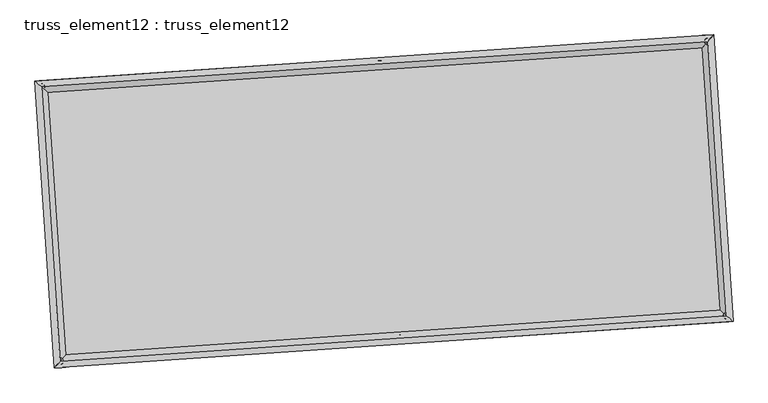
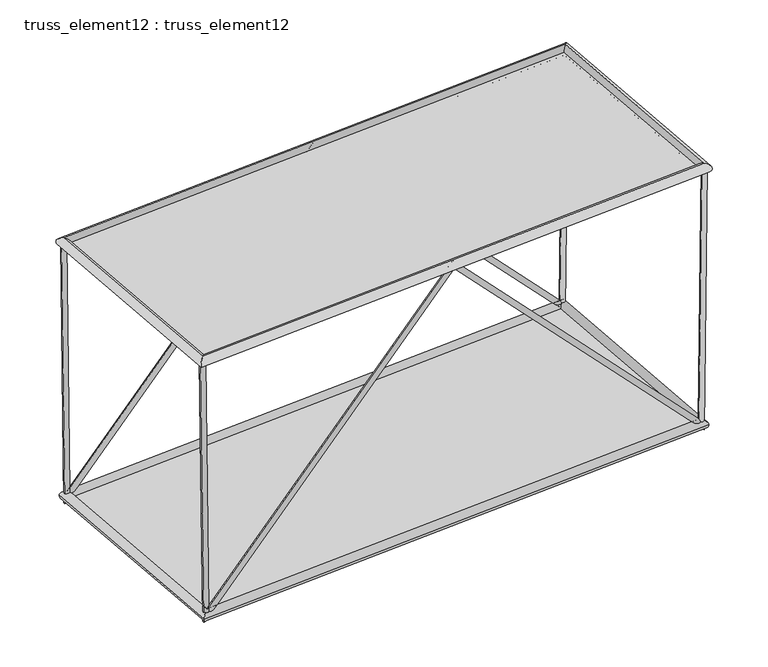
"""IFC4 building model written with IfcOpenShell, lengths in millimetres: plate geometry, truss_element12 : truss_element12."""

from ifc_helpers import new_model, si_unit, frame, origin, origin_with_axes, place, context, project, spatial, polyline, circle_curve, ellipse_curve, outline, extrude, source, transform, mapped, element, save
from ifc_brep_helpers import plane_surface, cylinder_surface, advanced_brep


def truss_element12_truss_element12_2c86acb7(model_context):
    return source(origin(), model_context, "Body", "SolidModel", [
        advanced_brep(
        [(-3728.3550112, 2271.9000693, 5000.230225), (-3827.45033, 2258.5393422, 4998.9618576), (-3666.4925131, 2276.1182379, 122.5885244), (-3762.4943697, 2262.9684422, -122.5885244), (1063.1473442, 2598.6144007, 5071.7241818), (1063.6040901, 2592.0417504, 4927.4822409), (5793.903749, 2921.1866967, 122.5964773), (5890.857228, 2921.1937918, -122.5964773), (5854.658099, 2925.3293049, 5000.2332074), (5954.6501108, 2925.543586, 4998.9875555)],
        [
            (0, 1, circle_curve(frame((-3777.9026706, 2265.2197058, 4999.5960413), z_axis=(-0.012681845830498275, -0.0008647268589742656, 0.9999192082532422), x_axis=(-0.13360744533254773, 0.991033979828119, -0.0008374829847137765)), 50.0)),
            (1, 0, circle_curve(frame((-3777.9026706, 2265.2197058, 4999.5960413), z_axis=(-0.012681845830498275, -0.0008647268589742656, 0.9999192082532422), x_axis=(-0.13360744533254773, 0.991033979828119, -0.0008374829847137765)), 50.0)),
            (0, 2),
            (2, 3, ellipse_curve(frame((-3714.4934414, 2269.54334, 0.0), z_axis=(-0.9281379125811652, -0.06328619607639939, 0.3668172196280557), x_axis=(0.36596744941726267, 0.02495392920324594, 0.9302930330730971)), 132.0610358, 50.0)),
            (3, 1),
            (3, 2, ellipse_curve(frame((-3714.4934414, 2269.54334, 0.0), z_axis=(-0.9281379125811652, -0.06328619607639939, 0.3668172196280557), x_axis=(0.36596744941726267, 0.02495392920324594, 0.9302930330730971)), 132.0610358, 50.0)),
            (2, 4),
            (4, 5, ellipse_curve(frame((1063.3757172, 2595.3280756, 4999.6032114), z_axis=(-0.99768339431723, -0.068028238108855, -5.9358703528731525e-05), x_axis=(5.922119292306359e-05, 4.038068026292035e-06, -0.9999999982382721)), 72.2780144, 50.0)),
            (5, 3),
            (5, 4, ellipse_curve(frame((1063.3757172, 2595.3280756, 4999.6032114), z_axis=(-0.99768339431723, -0.068028238108855, -5.9358703528731525e-05), x_axis=(5.922119292306359e-05, 4.038068026292035e-06, -0.9999999982382721)), 72.2780144, 50.0)),
            (4, 6),
            (6, 7, ellipse_curve(frame((5842.3804885, 2921.1902443, 0.0), z_axis=(-0.9280745157714422, -0.06328187328893672, -0.3669783340861503), x_axis=(-0.3661281906369709, -0.02496488953598652, 0.9302294890570573)), 132.0786249, 50.0)),
            (7, 5),
            (7, 6, ellipse_curve(frame((5842.3804885, 2921.1902443, 0.0), z_axis=(-0.9280745157714422, -0.06328187328893672, -0.3669783340861503), x_axis=(-0.3661281906369709, -0.02496488953598652, 0.9302294890570573)), 132.0786249, 50.0)),
            (8, 9, circle_curve(frame((5904.6541049, 2925.4364454, 4999.6103815), z_axis=(0.012454723282468173, 0.0008492402357941579, 0.9999220762934375), x_axis=(-0.002153222592044798, 0.9999973435725115, -0.0008224842793232085)), 50.0)),
            (9, 8, circle_curve(frame((5904.6541049, 2925.4364454, 4999.6103815), z_axis=(0.012454723282468173, 0.0008492402357941579, 0.9999220762934375), x_axis=(-0.002153222592044798, 0.9999973435725115, -0.0008224842793232085)), 50.0)),
            (6, 8),
            (9, 7),
        ],
        [
            plane_surface(frame((-3777.9026706, 2315.2196871, 4999.6392811), z_axis=(-0.012681845830499536, -0.000864726858973905, 0.9999192082532424), x_axis=(0.9999195821596513, -1.0967214670642997e-05, 0.012681841088294742))),
            cylinder_surface(frame((-3777.9026706, 2265.2197058, 4999.5960413), z_axis=(-0.012681845830498278, -0.0008647268589742659, 0.9999192082532424), x_axis=(-0.13360744533254773, 0.991033979828119, -0.0008374829847137765)), 50.0),
            cylinder_surface(frame((-3714.4934414, 2269.54334, 0.0), z_axis=(-0.6901279623524452, -0.04705720233082468, -0.7221558109494499), x_axis=(-0.020411445780293115, 0.9987523847393089, -0.04557462955089897)), 50.0),
            cylinder_surface(frame((1063.3757172, 2595.3280756, 4999.6032114), z_axis=(-0.6902134913462256, -0.04706303422778687, 0.7220736854178583), x_axis=(-0.11534401236489931, 0.9922792938963748, -0.04558027770953044)), 50.0),
            plane_surface(frame((5904.6541049, 2875.4364635, 4999.6528468), z_axis=(0.012454723282466664, 0.0008492402357928526, 0.9999220762934377), x_axis=(0.9999224369259634, -1.0577872590289415e-05, -0.012454718790539939))),
            cylinder_surface(frame((5842.3804885, 2921.1902443, 0.0), z_axis=(-0.012454723282468173, -0.0008492402357941579, -0.9999220762934375), x_axis=(-0.002153222592044798, 0.9999973435725115, -0.0008224842793232085)), 50.0),
        ],
        [
            (0, [[1, 2]]),
            (1, [[-1, 3, 4, 5]]),
            (1, [[-2, -5, 6, -3]]),
            (2, [[-4, 7, 8, 9]]),
            (2, [[-6, -9, 10, -7]]),
            (3, [[-8, 11, 12, 13]]),
            (3, [[-10, -13, 14, -11]]),
            (4, [[15, 16]]),
            (5, [[-12, 17, -16, 18]]),
            (5, [[-14, -18, -15, -17]]),
        ],
    ),
        advanced_brep(
        [(-3456.2420582, -1718.833515, 5000.230225), (-3555.3373771, -1732.1942421, 4998.9618576), (-3394.3795602, -1714.6153464, 122.5885244), (-3490.3814168, -1727.7651421, -122.5885244), (1335.2602971, -1392.1191836, 5071.7241818), (1335.7170431, -1398.6918339, 4927.4822409), (6066.016702, -1069.5468876, 122.5964773), (6162.9701809, -1069.5397925, -122.5964773), (6126.7710519, -1065.4042794, 5000.2332074), (6226.7630638, -1065.1899983, 4998.9875555)],
        [
            (0, 1, circle_curve(frame((-3505.7897177, -1725.5138785, 4999.5960413), z_axis=(-0.012681845830497715, -0.0008647268589742125, 0.9999192082532423), x_axis=(-0.13360744533254784, 0.991033979828119, -0.0008374829847137556)), 50.0)),
            (1, 0, circle_curve(frame((-3505.7897177, -1725.5138785, 4999.5960413), z_axis=(-0.012681845830497715, -0.0008647268589742125, 0.9999192082532423), x_axis=(-0.13360744533254784, 0.991033979828119, -0.0008374829847137556)), 50.0)),
            (0, 2),
            (2, 3, ellipse_curve(frame((-3442.3804885, -1721.1902443, 0.0), z_axis=(-0.9281379125811646, -0.06328619607639936, 0.36681721962805663), x_axis=(0.3659674494172635, 0.02495392920324602, 0.930293033073097)), 132.0610358, 50.0)),
            (3, 1),
            (3, 2, ellipse_curve(frame((-3442.3804885, -1721.1902443, 0.0), z_axis=(-0.9281379125811646, -0.06328619607639936, 0.36681721962805663), x_axis=(0.3659674494172635, 0.02495392920324602, 0.930293033073097)), 132.0610358, 50.0)),
            (2, 4),
            (4, 5, ellipse_curve(frame((1335.4886701, -1395.4055087, 4999.6032114), z_axis=(-0.9976833943172299, -0.06802823810885503, -5.935870352808952e-05), x_axis=(5.922119292244865e-05, 4.03806802626321e-06, -0.9999999982382721)), 72.2780144, 50.0)),
            (5, 3),
            (5, 4, ellipse_curve(frame((1335.4886701, -1395.4055087, 4999.6032114), z_axis=(-0.9976833943172299, -0.06802823810885503, -5.935870352808952e-05), x_axis=(5.922119292244865e-05, 4.03806802626321e-06, -0.9999999982382721)), 72.2780144, 50.0)),
            (4, 6),
            (6, 7, ellipse_curve(frame((6114.4934414, -1069.54334, 0.0), z_axis=(-0.928074515771442, -0.06328187328893677, -0.3669783340861506), x_axis=(-0.3661281906369714, -0.024964889535986565, 0.9302294890570572)), 132.0786249, 50.0)),
            (7, 5),
            (7, 6, ellipse_curve(frame((6114.4934414, -1069.54334, 0.0), z_axis=(-0.928074515771442, -0.06328187328893677, -0.3669783340861506), x_axis=(-0.3661281906369714, -0.024964889535986565, 0.9302294890570572)), 132.0786249, 50.0)),
            (8, 9, circle_curve(frame((6176.7670578, -1065.2971389, 4999.6103815), z_axis=(0.012454723282467507, 0.0008492402357941209, 0.9999220762934375), x_axis=(-0.0021532225920447086, 0.9999973435725115, -0.0008224842793231741)), 50.0)),
            (9, 8, circle_curve(frame((6176.7670578, -1065.2971389, 4999.6103815), z_axis=(0.012454723282467507, 0.0008492402357941209, 0.9999220762934375), x_axis=(-0.0021532225920447086, 0.9999973435725115, -0.0008224842793231741)), 50.0)),
            (6, 8),
            (9, 7),
        ],
        [
            plane_surface(frame((-3505.7897177, -1675.5138972, 4999.6392811), z_axis=(-0.012681845830499536, -0.000864726858973898, 0.9999192082532424), x_axis=(0.9999195821596513, -1.0967214670642997e-05, 0.012681841088294742))),
            cylinder_surface(frame((-3505.7897177, -1725.5138785, 4999.5960413), z_axis=(-0.012681845830497715, -0.0008647268589742125, 0.9999192082532423), x_axis=(-0.13360744533254784, 0.991033979828119, -0.0008374829847137556)), 50.0),
            cylinder_surface(frame((-3442.3804885, -1721.1902443, 0.0), z_axis=(-0.6901279623524461, -0.047057202330824756, -0.722155810949449), x_axis=(-0.020411445780293143, 0.9987523847393089, -0.045574629550899075)), 50.0),
            cylinder_surface(frame((1335.4886701, -1395.4055087, 4999.6032114), z_axis=(-0.6902134913462256, -0.047063034227786904, 0.7220736854178583), x_axis=(-0.11534401236489945, 0.9922792938963748, -0.045580277709530506)), 50.0),
            plane_surface(frame((6176.7670578, -1115.2971208, 4999.6528468), z_axis=(0.012454723282466664, 0.0008492402357928471, 0.9999220762934377), x_axis=(0.9999224369259634, -1.0577872589401237e-05, -0.012454718790539939))),
            cylinder_surface(frame((6114.4934414, -1069.54334, 0.0), z_axis=(-0.012454723282467507, -0.0008492402357941209, -0.9999220762934375), x_axis=(-0.0021532225920447086, 0.9999973435725115, -0.0008224842793231741)), 50.0),
        ],
        [
            (0, [[1, 2]]),
            (1, [[-1, 3, 4, 5]]),
            (1, [[-2, -5, 6, -3]]),
            (2, [[-4, 7, 8, 9]]),
            (2, [[-6, -9, 10, -7]]),
            (3, [[-8, 11, 12, 13]]),
            (3, [[-10, -13, 14, -11]]),
            (4, [[15, 16]]),
            (5, [[-12, 17, -16, 18]]),
            (5, [[-14, -18, -15, -17]]),
        ],
    ),
        advanced_brep(
        [(-3505.7859545, -1725.5097077, 4909.5960414), (-3505.7934808, -1725.5180494, 5089.5960412), (-3777.906965, 2265.2233272, 5089.5960412), (-3777.8983761, 2265.2160844, 4909.5960414), (5904.6576027, 2925.4405981, 5089.6103814), (5904.6506071, 2925.4322927, 4909.6103815), (6176.7710869, -1065.3007784, 5089.6103814), (6176.7630287, -1065.2934994, 4909.6103815)],
        [
            (0, 1, ellipse_curve(frame((-3505.7897177, -1725.5138785, 4999.5960413), z_axis=(-0.7535719234046869, 0.6573654662781344, -1.0448234971291915e-06), x_axis=(-0.6573654662773117, -0.7535719234054046, -1.0448235032548692e-06)), 127.2792206, 90.0)),
            (1, 2),
            (2, 3, ellipse_curve(frame((-3777.9026706, 2265.2197058, 4999.5960413), z_axis=(-0.6573654662773116, -0.7535719234054046, -1.0448235045172827e-06), x_axis=(0.7535719234046869, -0.6573654662781343, 1.0448234983916052e-06)), 127.2792206, 90.0)),
            (3, 0),
            (1, 0, ellipse_curve(frame((-3505.7897177, -1725.5138785, 4999.5960413), z_axis=(-0.7535719234046869, 0.6573654662781344, -1.0448234971291915e-06), x_axis=(-0.6573654662773117, -0.7535719234054046, -1.0448235032548692e-06)), 127.2792206, 90.0)),
            (3, 2, ellipse_curve(frame((-3777.9026706, 2265.2197058, 4999.5960413), z_axis=(-0.6573654662773116, -0.7535719234054046, -1.0448235045172827e-06), x_axis=(0.7535719234046869, -0.6573654662781343, 1.0448234983916052e-06)), 127.2792206, 90.0)),
            (2, 4),
            (4, 5, ellipse_curve(frame((5904.6541049, 2925.4364454, 4999.6103815), z_axis=(-0.7535719234046876, 0.6573654662781336, -1.0448234953288471e-06), x_axis=(-0.6573654662773109, -0.7535719234054052, -1.0448235075800405e-06)), 127.2792206, 90.0)),
            (5, 3),
            (5, 4, ellipse_curve(frame((5904.6541049, 2925.4364454, 4999.6103815), z_axis=(-0.7535719234046876, 0.6573654662781336, -1.0448234953288471e-06), x_axis=(-0.6573654662773109, -0.7535719234054052, -1.0448235075800405e-06)), 127.2792206, 90.0)),
            (4, 6),
            (6, 7, ellipse_curve(frame((6176.7670578, -1065.2971389, 4999.6103815), z_axis=(0.657365466277311, 0.753571923405405, 1.044823506317627e-06), x_axis=(-0.7535719234046873, 0.6573654662781341, -1.0448234940664328e-06)), 127.2792206, 90.0)),
            (7, 5),
            (7, 6, ellipse_curve(frame((6176.7670578, -1065.2971389, 4999.6103815), z_axis=(0.657365466277311, 0.753571923405405, 1.044823506317627e-06), x_axis=(-0.7535719234046873, 0.6573654662781341, -1.0448234940664328e-06)), 127.2792206, 90.0)),
            (6, 1),
            (0, 7),
        ],
        [
            cylinder_surface(frame((-3505.7897177, -1725.5138785, 4999.5960413), z_axis=(0.06802823822869937, -0.9976833960748767, 0.0), x_axis=(-0.997683395070632, -0.06802823816022374, -4.486817461283446e-05)), 90.0),
            cylinder_surface(frame((-3777.9026706, 2265.2197058, 4999.5960413), z_axis=(-0.9976833960737876, -0.06802823822862634, -1.47760356604302e-06), x_axis=(-0.06802823810069528, 0.9976833951400482, -4.339057104385098e-05)), 90.0),
            cylinder_surface(frame((5904.6541049, 2925.4364454, 4999.6103815), z_axis=(-0.06802823822870101, 0.9976833960748767, 0.0), x_axis=(0.997683395198563, 0.06802823816894851, -4.19129674878619e-05)), 90.0),
            cylinder_surface(frame((6176.7670578, -1065.2971389, 4999.6103815), z_axis=(0.9976833960737875, 0.06802823822862625, 1.4776035642576973e-06), x_axis=(0.06802823822862625, -0.997683395131325, -4.339057105939159e-05)), 90.0),
        ],
        [
            (0, [[1, 2, 3, 4]]),
            (0, [[5, -4, 6, -2]]),
            (1, [[-3, 7, 8, 9]]),
            (1, [[-6, -9, 10, -7]]),
            (2, [[-8, 11, 12, 13]]),
            (2, [[-10, -13, 14, -11]]),
            (3, [[-12, 15, -1, 16]]),
            (3, [[-14, -16, -5, -15]]),
        ],
    ),
        advanced_brep(
        [(-3358.7115243, -1625.2761972, 0.0), (-3526.0494527, -1817.1042913, 0.0), (-3810.4074885, 2353.2123043, 0.0), (-3618.5793943, 2185.8743758, 0.0), (5926.0494527, 3017.1042913, 0.0), (5758.7115243, 2825.2761972, 0.0), (6210.4074885, -1153.2123043, 0.0), (6018.5793943, -985.8743758, 0.0)],
        [
            (0, 1, ellipse_curve(frame((-3442.3804885, -1721.1902443, 0.0), z_axis=(-0.753571923405458, 0.6573654662780806, 0.0), x_axis=(-0.6573654662780806, -0.753571923405458, 0.0)), 127.2792206, 90.0)),
            (1, 2),
            (2, 3, ellipse_curve(frame((-3714.4934414, 2269.54334, 0.0), z_axis=(-0.6573654662780806, -0.753571923405458, 0.0), x_axis=(0.7535719234054579, -0.6573654662780809, 0.0)), 127.2792206, 90.0)),
            (3, 0),
            (1, 0, ellipse_curve(frame((-3442.3804885, -1721.1902443, 0.0), z_axis=(-0.753571923405458, 0.6573654662780806, 0.0), x_axis=(-0.6573654662780806, -0.753571923405458, 0.0)), 127.2792206, 90.0)),
            (3, 2, ellipse_curve(frame((-3714.4934414, 2269.54334, 0.0), z_axis=(-0.6573654662780806, -0.753571923405458, 0.0), x_axis=(0.7535719234054579, -0.6573654662780809, 0.0)), 127.2792206, 90.0)),
            (2, 4),
            (4, 5, ellipse_curve(frame((5842.3804885, 2921.1902443, 0.0), z_axis=(-0.7535719234054586, 0.6573654662780799, 0.0), x_axis=(-0.6573654662780801, -0.7535719234054584, 0.0)), 127.2792206, 90.0)),
            (5, 3),
            (5, 4, ellipse_curve(frame((5842.3804885, 2921.1902443, 0.0), z_axis=(-0.7535719234054586, 0.6573654662780799, 0.0), x_axis=(-0.6573654662780801, -0.7535719234054584, 0.0)), 127.2792206, 90.0)),
            (4, 6),
            (6, 7, ellipse_curve(frame((6114.4934414, -1069.54334, 0.0), z_axis=(0.6573654662780799, 0.7535719234054586, 0.0), x_axis=(-0.7535719234054586, 0.6573654662780799, 0.0)), 127.2792206, 90.0)),
            (7, 5),
            (7, 6, ellipse_curve(frame((6114.4934414, -1069.54334, 0.0), z_axis=(0.6573654662780799, 0.7535719234054586, 0.0), x_axis=(-0.7535719234054586, 0.6573654662780799, 0.0)), 127.2792206, 90.0)),
            (6, 1),
            (0, 7),
        ],
        [
            cylinder_surface(frame((-3442.3804885, -1721.1902443, 0.0), z_axis=(0.06802823822870088, -0.9976833960748768, 0.0), x_axis=(-0.9976833960748768, -0.06802823822870088, 0.0)), 90.0),
            cylinder_surface(frame((-3714.4934414, 2269.54334, 0.0), z_axis=(-0.9976833960748767, -0.06802823822870208, 0.0), x_axis=(-0.06802823822870208, 0.9976833960748767, 0.0)), 90.0),
            cylinder_surface(frame((5842.3804885, 2921.1902443, 0.0), z_axis=(-0.06802823822870274, 0.9976833960748765, 0.0), x_axis=(0.9976833960748765, 0.06802823822870274, 0.0)), 90.0),
            cylinder_surface(frame((6114.4934414, -1069.54334, 0.0), z_axis=(0.9976833960748767, 0.06802823822870205, 0.0), x_axis=(0.06802823822870205, -0.9976833960748767, 0.0)), 90.0),
        ],
        [
            (0, [[1, 2, 3, 4]]),
            (0, [[5, -4, 6, -2]]),
            (1, [[-3, 7, 8, 9]]),
            (1, [[-6, -9, 10, -7]]),
            (2, [[-8, 11, 12, 13]]),
            (2, [[-10, -13, 14, -11]]),
            (3, [[-12, 15, -1, 16]]),
            (3, [[-14, -16, -5, -15]]),
        ],
    ),
        extrude(outline(polyline([(-3442.3804885, -1721.1902443), (-3714.4934414, 2269.54334), (5842.3804885, 2921.1902443), (6114.4934414, -1069.54334), (-3442.3804885, -1721.1902443)])), origin_with_axes(), (0.0, 0.0, 1.0), 20.0),
        extrude(outline(polyline([(-1999.9999999, 4852.5197541), (2000.0000001, 4852.5197541), (2000.0, -4852.5197541), (-2000.0, -4852.5197541), (-1999.9999999, 4852.5197541)])), frame((1199.4321936, 599.9612834, 4999.6032114), z_axis=(-1.474180543527448e-06, -1.0051877171978412e-07, 0.9999999999989084), x_axis=(-0.06802823822870088, 0.9976833960748767, 0.0)), (0.0, 0.0, 1.0), 20.0),
    ])


if __name__ == "__main__":
    model = new_model("IFC4")
    model_context = context("Model", 3, world=origin())
    ifc_project = project(units=[si_unit("LENGTHUNIT", "METRE", prefix="MILLI")], contexts=[model_context])
    site = spatial("IfcSite", under=ifc_project)
    building = spatial("IfcBuilding", under=site)
    placement = place(None, origin())
    truss_element12_truss_element12_shape = truss_element12_truss_element12_2c86acb7(model_context)
    element("IfcPlate", 1, ObjectType="truss_element12 : truss_element12", at=placement, inside=building, context=model_context, shape_type="MappedRepresentation", body=[
        mapped(truss_element12_truss_element12_shape, transform((0.0, 0.0, 0.0), x_axis=(1.0, 0.0, 0.0), y_axis=(0.0, 1.0, 0.0), z_axis=(0.0, 0.0, 1.0))),
    ])
    save(model, "model.ifc")

# Revit data of these elements
# Type "truss_element12 : truss_element12"
#   steellbar1 = 90 mm
#   steelbar2 = 50 mm
#   offset1 = 5000 mm
#   M = Default Roof
# Element 1 (IfcPlate, "truss_element12 : truss_element12")
#   Materials on its faces: "Default Roof"
# Materials
#   "Default Roof": class "Miscellaneous", colour RGB 0 127 0, transparency 0, Comments = "Rendering appearance not upgraded Rendering appearance not upgraded ", Cost = 0
